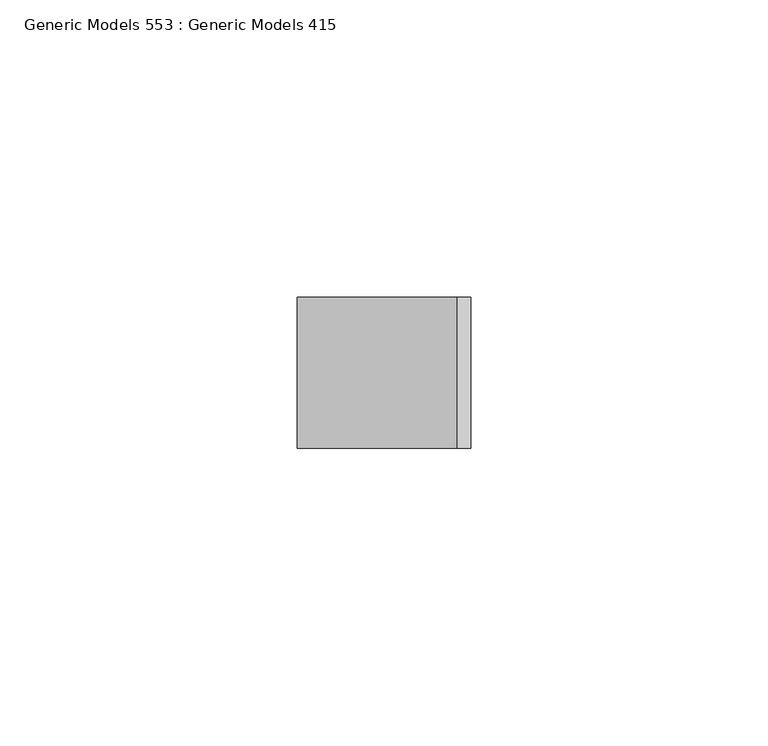
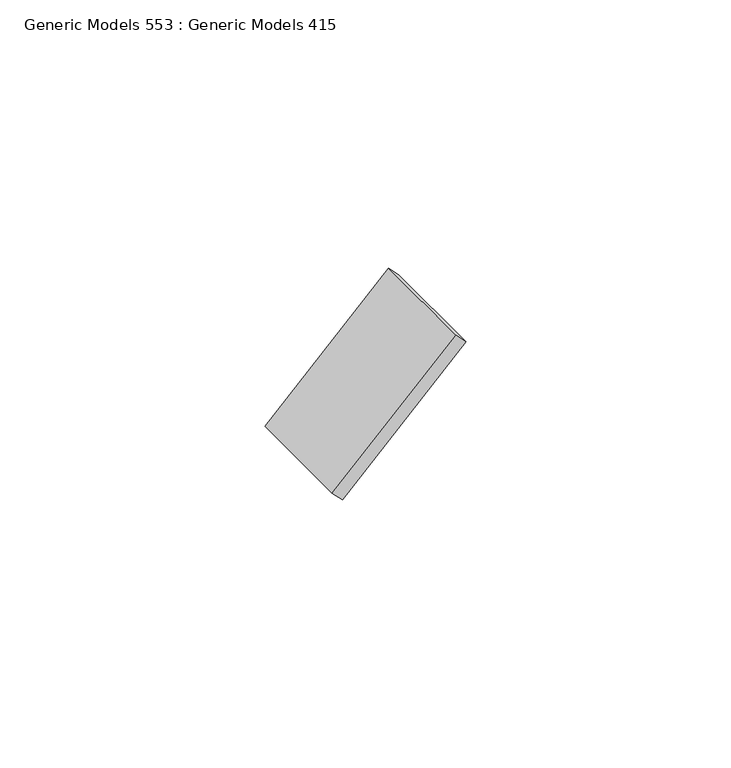
"""IFC4 building model written with IfcOpenShell, lengths in millimetres: proxy geometry, Generic Models 553 : Generic Models 415."""

from ifc_helpers import new_model, si_unit, frame, origin, place, context, project, spatial, polyline, outline, extrude, source, transform, mapped, element, save


def generic_models_553_generic_models_415_9c1bf2ed(model_context):
    return source(origin(), model_context, "Body", "SweptSolid", [
        extrude(outline(polyline([(0.0, -3.175), (0.0, 0.0), (25.4, 0.0), (25.4, -3.175), (0.0, -3.175)])), frame((7848.0411784, 4501.3863946, 124622.8849742), z_axis=(0.7071067811867181, 0.0, 0.707106781186377), x_axis=(0.0, -1.0, 0.0)), (0.0, 0.0, 1.0), 38.1),
    ])


if __name__ == "__main__":
    model = new_model("IFC4")
    model_context = context("Model", 3, world=origin())
    ifc_project = project(units=[si_unit("LENGTHUNIT", "METRE", prefix="MILLI")], contexts=[model_context])
    site = spatial("IfcSite", under=ifc_project)
    building = spatial("IfcBuilding", under=site)
    placement = place(None, origin())
    generic_models_553_generic_models_415_shape = generic_models_553_generic_models_415_9c1bf2ed(model_context)
    element("IfcBuildingElementProxy", 1, Name="Generic Models 553 : Generic Models 415", ObjectType="Generic Models 553 : Generic Models 415", at=placement, inside=building, context=model_context, shape_type="MappedRepresentation", body=[
        mapped(generic_models_553_generic_models_415_shape, transform((0.0, 0.0, 0.0), x_axis=(1.0, 0.0, 0.0), y_axis=(0.0, 1.0, 0.0), z_axis=(0.0, 0.0, 1.0))),
    ])
    save(model, "model.ifc")

# Revit data of these elements
# Element 1 (IfcBuildingElementProxy, "Generic Models 553 : Generic Models 415")
#   Materials on its faces: "_WELDED STEEL TABS FOR LOUVER ATTACHMENT"
# Materials
#   "_WELDED STEEL TABS FOR LOUVER ATTACHMENT": class "Metal", colour RGB 199 199 199, transparency 0, Description = "Structural steel 50ksi", Cost = 0
